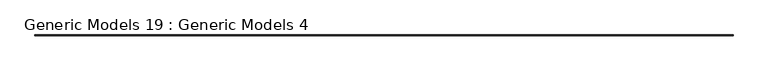
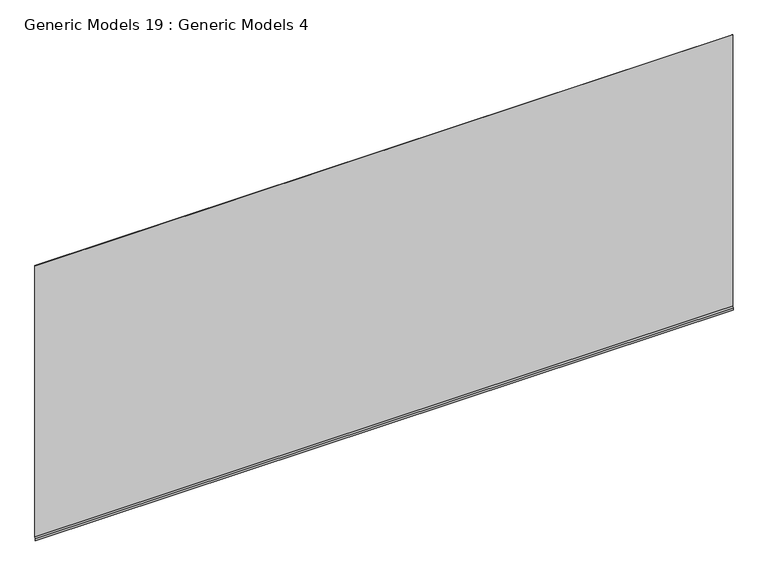
"""IFC4 building model written with IfcOpenShell, lengths in millimetres: proxy geometry, Generic Models 19 : Generic Models 4."""

from ifc_helpers import new_model, si_unit, frame, origin, place, context, project, spatial, polyline, outline, extrude, source, transform, mapped, element, save


def generic_models_19_generic_models_4_8315374a(model_context):
    return source(origin(), model_context, "Body", "SweptSolid", [
        extrude(outline(polyline([(-7075.0716353, 123876.8559884), (-7079.9031787, 123863.581432), (-7079.9031787, 123844.698879), (-7080.6969287, 123844.698879), (-7080.6969287, 123863.7213915), (-7075.8653853, 123876.9959479), (-7075.8653853, 126422.4981417), (-7075.0716353, 126422.4981417), (-7075.0716353, 123876.8559884)])), frame((2196.9263704, 0.0, 0.0), z_axis=(1.0, 0.0, 0.0), x_axis=(0.0, 1.0, 0.0)), (0.0, 0.0, 1.0), 6189.931498),
    ])


if __name__ == "__main__":
    model = new_model("IFC4")
    model_context = context("Model", 3, world=origin())
    ifc_project = project(units=[si_unit("LENGTHUNIT", "METRE", prefix="MILLI")], contexts=[model_context])
    site = spatial("IfcSite", under=ifc_project)
    building = spatial("IfcBuilding", under=site)
    placement = place(None, origin())
    generic_models_19_generic_models_4_shape = generic_models_19_generic_models_4_8315374a(model_context)
    element("IfcBuildingElementProxy", 1, Name="Generic Models 19 : Generic Models 4", ObjectType="Generic Models 19 : Generic Models 4", at=placement, inside=building, context=model_context, shape_type="MappedRepresentation", body=[
        mapped(generic_models_19_generic_models_4_shape, transform((0.0, 0.0, 0.0), x_axis=(1.0, 0.0, 0.0), y_axis=(0.0, 1.0, 0.0), z_axis=(0.0, 0.0, 1.0))),
    ])
    save(model, "model.ifc")

# Revit data of these elements
# Element 1 (IfcBuildingElementProxy, "Generic Models 19 : Generic Models 4")
#   Materials on its faces: "_(2) LAYERS NO. 30 ASTM D226 ASPHALT SATURATED ORGANIC FELT"
# Materials
#   "_(2) LAYERS NO. 30 ASTM D226 ASPHALT SATURATED ORGANIC FELT": class "Generic", colour RGB 67 154 161, transparency 0, Cost = 0
